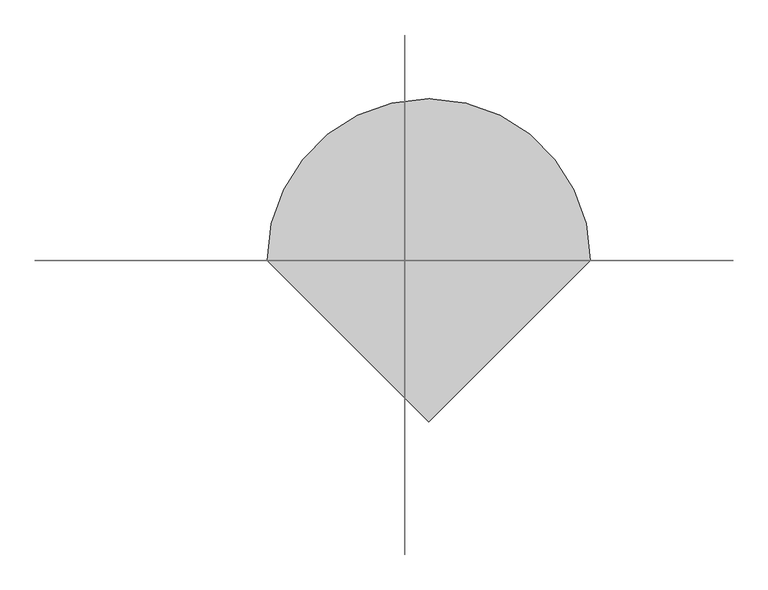
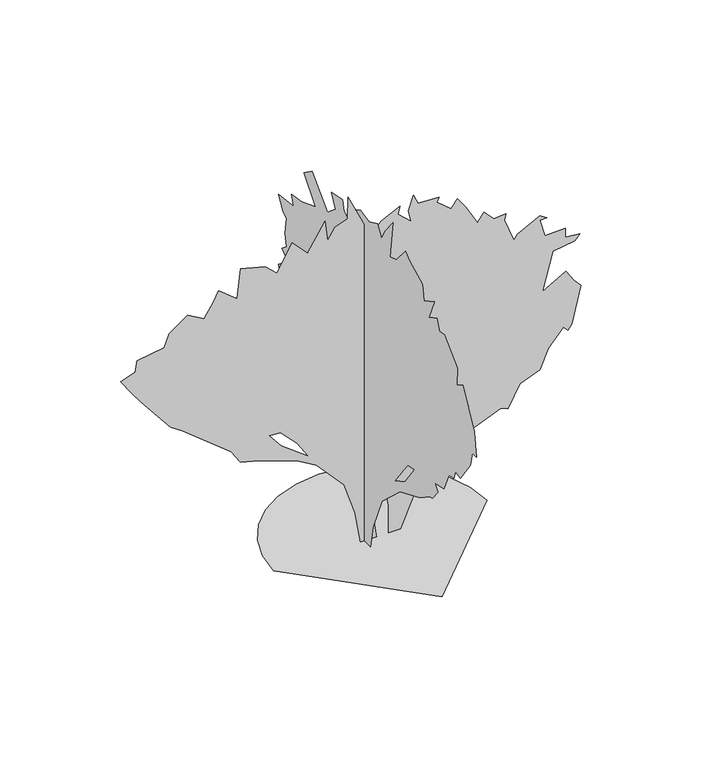
"""IFC4 building model written with IfcOpenShell, lengths in millimetres: proxy geometry, honey myrtle 26117 : honey myrtle 26117."""

from ifc_helpers import new_model, si_unit, origin, place, context, project, spatial, triangles, source, transform, mapped, element, save


def entourage_3ce3a2b3(model_context):
    return source(origin(), model_context, "Body", "Tessellation", [
        triangles([(-396.3767504, 0.0, 8.22e-05), (-385.8992649, 90.8237077, 8.22e-05), (-356.0543206, 174.2306261, 8.22e-05), (-309.2370838, 247.8313661, 8.22e-05), (-247.8313661, 309.2370838, 8.22e-05), (-174.2306261, 356.0543206, 8.22e-05), (-90.8237077, 385.8992649, 8.22e-05), (1.73e-05, 396.3767504, 8.22e-05), (90.8237077, 385.8992649, 8.22e-05), (174.2306261, 356.0543206, 8.22e-05), (247.8313661, 309.2370838, 8.22e-05), (309.2370838, 247.8313661, 8.22e-05), (356.0543206, 174.2306261, 8.22e-05), (385.8992649, 90.8237077, 8.22e-05), (396.3767504, -3.47e-05, 8.22e-05), (-5.2e-05, -396.3767504, 8.22e-05), (-59.3577095, 35.0059915, 9.26e-05), (-59.3577095, 44.8705806, 101.5460546), (-59.3577095, 75.4742449, 222.0478563), (-59.3577095, 168.9964434, 326.3007588), (-59.3577095, 285.8741748, 405.6706235), (-59.3579639, 459.2340692, 576.3228888), (-59.3579639, 503.9253456, 625.6344137), (-59.3579639, 553.1479589, 751.1941189), (-59.3579639, 491.6190474, 799.7715317), (-59.3579639, 530.478485, 828.915465), (-59.3579639, 501.3320083, 851.5849388), (-59.3579639, 511.0474763, 900.1598808), (-59.3579639, 501.3320083, 961.688756), (-59.3579639, 524.0014821, 977.8812269), (-59.3579639, 553.1479589, 1026.4561689), (-59.3579639, 455.9955677, 1039.4101748), (-59.3579639, 469.4956884, 1077.0376745), (-59.3579639, 404.1821606, 1087.9850441), (-59.3579639, 313.5068087, 1123.6085238), (-59.3579639, 387.9896896, 1211.0454105), (-59.3579639, 336.1762825, 1249.9048119), (-59.3579639, 235.7859349, 1149.5164627), (-59.3579639, 183.9712561, 1191.6144018), (-59.3579639, 209.8784683, 1243.4278816), (-59.3579639, 138.9198272, 1256.3183739), (-59.3579639, 128.9188388, 1217.5224134), (-59.3579639, 70.6279291, 1185.1373989), (-59.3579639, 83.5816624, 1253.143277), (-59.3579639, 25.4436618, 1284.1769932), (-59.3579639, -29.761912, 1272.5743584), (-59.3579639, -86.0073592, 1299.3586246), (-59.3579639, -110.7212849, 1256.3817421), (-59.3579639, -133.3899957, 1298.4822247), (-59.3579639, -185.2039207, 1363.2496376), (-59.3577095, -165.7739475, 1217.5224134), (-59.3577095, -207.8728858, 1230.4738758), (-59.3577095, -266.3644464, 1299.9199276), (-59.3577095, -292.0717617, 1279.0512886), (-59.3577095, -376.2676217, 1236.950806), (-59.3577095, -385.9830897, 1178.660396), (-59.3577095, -450.7505027, 1214.2838757), (-59.3577095, -418.3680679, 1133.3239918), (-59.3577095, -466.9429736, 1159.22946), (-59.3577095, -484.2835213, 1117.1086298), (-59.3577095, -515.5204227, 1123.6085238), (-59.3577095, -599.7162646, 1042.6486399), (-59.3577095, -596.4777632, 974.6427618), (-59.3577095, -635.3397079, 997.3122356), (-59.3577095, -709.8225889, 858.0619417), (-59.3577095, -722.7765947, 767.3865898), (-59.3577095, -696.8686558, 767.3865898), (-59.3577095, -683.91465, 712.3346449), (-59.3577095, -619.147237, 621.659293), (-59.3577095, -586.7622588, 628.1362959), (-59.3577095, -577.0493342, 595.7513177), (-59.3577095, -544.664356, 589.2743148), (-59.3577095, -512.2819213, 514.7914338), (-59.3577095, -453.9890041, 501.8400078), (-59.3577095, -473.4199765, 479.1705339), (-59.3577095, -438.083507, 433.2245012), (-59.3577095, -424.8450708, 430.5955919), (-59.3577095, -359.671251, 388.3935531), (-59.3577095, -230.5626891, 332.9860339), (-59.3577095, -112.6590482, 224.7923109), (-59.3577095, -55.1474106, 87.2636415), (-59.3577095, -39.476642, 8.38e-05), (-59.3577095, 5.8605105, 135.9018064), (-59.3577095, 2.7896791, 186.1833303), (-59.3577095, 12.337225, 304.2967785), (-59.3577095, 38.2442317, 288.1068329), (-59.3577095, 54.4362076, 262.1988576), (-59.3577095, 151.5875587, 349.6357444), (-59.3577095, 177.4947618, 469.4550296), (-59.3577095, 258.4549001, 547.176412), (-59.3577095, 255.2163986, 508.3169744), (-59.3577095, 226.0704487, 394.9721486), (-59.3577095, 255.2163986, 404.687653), (-59.3577095, 297.3143196, 550.4149135), (-59.3577095, 337.517407, 606.5056758), (-59.3577095, 326.4607781, 505.0785092), (-59.3577095, 307.0298058, 462.9780267), (-59.3577095, 358.8432129, 501.8400078), (-59.3579639, 368.5587173, 641.0903017), (-59.3579639, 410.6591635, 689.6651711), (-59.3579639, 410.6591635, 628.1362959), (-59.3577095, -198.157654, 356.112711), (-59.3577095, -261.769596, 391.7057055), (-59.3577095, -324.4541782, 475.9320325), (-59.3577095, -282.3562755, 469.4550296), (-59.3577095, -253.2100531, 430.5955919), (-267.2940953, -2.61e-05, 404.687653), (-308.6096875, -2.21e-05, 471.3142911), (-370.9208914, -1.84e-05, 534.2224425), (-413.0213739, -1.82e-05, 537.4609076), (-368.4215527, -2.15e-05, 482.1804156), (30.6369404, -5.02e-05, 0.0), (31.1304627, -4.38e-05, 108.1619844), (9.0696959, -3.61e-05, 237.4841779), (-47.0839311, -3.05e-05, 330.2047357), (-39.4309189, -4.01e-05, 170.4041154), (-14.7000316, -5.02e-05, 0.0), (-72.990889, -5.02e-05, 0.0), (-92.9872747, -4.29e-05, 122.5858678), (-134.4006626, -3.55e-05, 247.1552083), (-236.0793036, -2.88e-05, 358.7517941), (-302.2063538, -2.64e-05, 398.8659516), (-451.8807753, -2.32e-05, 453.2625587), (-519.8892331, -2.22e-05, 469.4550296), (-555.510133, -1.89e-05, 524.5069382), (-736.858366, -1.03e-05, 670.234235), (-778.9587759, -8.5e-06, 699.3807117), (-889.0625931, -4e-07, 835.3924679), (-924.6860727, 2.5e-06, 883.9674099), (-965.6003632, 6e-06, 942.4685629), (-911.7320669, 7.1e-06, 961.688756), (-905.255064, 9.6e-06, 1003.7892385), (-804.8642441, 1.06e-05, 1019.979166), (-785.4357788, 1.35e-05, 1068.5565788), (-717.4299007, 1.64e-05, 1117.1315208), (-655.8984821, 1.43e-05, 1081.5105846), (-620.2775459, 1.75e-05, 1136.5625296), (-600.8465735, 1.97e-05, 1172.1833931), (-532.8406591, 1.64e-05, 1117.1315208), (-519.8892331, 2.31e-05, 1230.4738758), (-429.2138449, 2.18e-05, 1207.8068727), (-383.8748972, 1.93e-05, 1165.7064629), (-328.8229886, 2.53e-05, 1266.0972828), (-270.5325967, 2.16e-05, 1204.5684076), (-205.7644389, 2.78e-05, 1308.1951492), (-196.0496976, 2.29e-05, 1227.2378815), (-167.6639666, 2.55e-05, 1270.8241745), (-121.5665623, 2.66e-05, 1288.7668293), (-119.7654549, 3.15e-05, 1371.5986919), (-34.1304544, 2.06e-05, 1188.3759367), (2.3015577, 2.34e-05, 1235.4267712), (72.7363851, 2.54e-05, 1269.3357479), (66.2596456, 2.37e-05, 1240.1892712), (114.8353143, 2.1e-05, 1194.8529396), (105.1200825, 2.37e-05, 1240.1892712), (124.5505553, 2.7e-05, 1295.2437595), (140.7425266, 2.47e-05, 1256.3817421), (218.4636638, 2.45e-05, 1253.143277), (211.1367854, 2.35e-05, 1235.7950626), (263.8015941, 2.08e-05, 1191.6144018), (286.4685245, 2.27e-05, 1223.9994164), (318.8535027, 2e-05, 1178.660396), (360.9514054, 1.56e-05, 1104.177515), (385.0814006, 1.75e-05, 1135.7446289), (422.4828604, 1.52e-05, 1097.7005121), (467.8192646, 1.54e-05, 1100.9390499), (461.3422617, 1.41e-05, 1078.2721195), (496.9657413, 8.7e-06, 987.5967676), (509.9172037, 9.8e-06, 1007.0277037), (594.1155527, 1.23e-05, 1049.1256428), (620.0235643, 1.14e-05, 1032.9331718), (593.290058, 1.13e-05, 1031.1069025), (613.5465614, 7.3e-06, 964.9272211), (688.0294424, 7.5e-06, 968.1657589), (688.0294424, 5.4e-06, 932.5448227), (743.0813147, 5e-06, 926.0678198), (723.6503786, 3.8e-06, 906.6368837), (642.6904947, 3.1e-06, 893.6828779), (603.8310571, -5.6e-06, 747.9555811), (691.2679075, -2.7e-06, 796.5330666), (720.4118408, -5.4e-06, 751.1941189), (746.3198524, -7.2e-06, 722.0501856), (713.9348379, -1.55e-05, 582.7973482), (697.7449104, -1.66e-05, 563.3688829), (681.5524395, -1.57e-05, 579.5613902), (626.5005672, -1.93e-05, 518.0299353), (594.1155527, -2.38e-05, 443.5470543), (519.6326717, -2.55e-05, 414.403121), (474.2962675, -3.03e-05, 333.4432371), (448.3882922, -2.98e-05, 343.1587415), (311.7719945, -3.3e-05, 288.0331637), (205.1723602, -3.7e-05, 221.2502851), (125.3034072, -4.32e-05, 117.1220752), (75.9746277, -5.02e-05, 0.0), (30.6369404, -3.34e-05, 281.62983), (43.5909303, -2.72e-05, 385.2566442), (7.9686832, -2.28e-05, 459.7395252), (-30.8919575, -2.45e-05, 430.5955919), (-38.6976243, -2.72e-05, 386.112624), (-2.6646859, -3.14e-05, 315.8842435), (150.4575132, -3.75e-05, 213.6229345), (215.0437962, -3.57e-05, 242.9182394), (296.5269221, -3.01e-05, 337.5199505), (331.8074721, -2.65e-05, 398.2106501), (278.0814637, -2.79e-05, 375.0661689), (195.3344433, -3.11e-05, 320.3901821), (154.7673882, -3.52e-05, 251.8887493)], [[16, 15, 1], [15, 14, 1], [1, 14, 2], [14, 13, 2], [2, 13, 3], [3, 13, 4], [13, 12, 4], [12, 11, 4], [4, 11, 5], [5, 11, 6], [6, 11, 7], [7, 11, 8], [8, 11, 9], [9, 11, 10], [90, 93, 91], [91, 93, 92], [93, 90, 94], [98, 95, 99], [17, 83, 18], [95, 98, 96], [50, 49, 51], [57, 56, 58], [85, 88, 86], [49, 48, 51], [84, 102, 85], [18, 83, 19], [83, 87, 19], [31, 30, 32], [19, 87, 20], [40, 39, 41], [41, 39, 42], [26, 25, 27], [30, 29, 32], [17, 82, 83], [82, 81, 83], [81, 80, 83], [83, 80, 84], [84, 80, 102], [80, 79, 102], [102, 79, 103], [79, 78, 103], [103, 78, 104], [78, 77, 104], [33, 32, 34], [66, 65, 67], [59, 58, 60], [36, 35, 37], [37, 35, 38], [86, 88, 87], [87, 88, 20], [88, 92, 20], [20, 92, 21], [92, 93, 21], [93, 97, 21], [21, 97, 22], [64, 63, 65], [53, 52, 54], [47, 46, 48], [75, 74, 76], [24, 23, 25], [44, 43, 45], [45, 43, 46], [96, 98, 97], [97, 98, 22], [98, 101, 22], [22, 101, 23], [23, 101, 25], [101, 100, 25], [69, 68, 70], [76, 74, 77], [77, 74, 104], [71, 70, 72], [88, 85, 89], [85, 102, 89], [102, 106, 89], [106, 105, 89], [54, 52, 55], [55, 52, 56], [61, 60, 62], [62, 60, 63], [42, 39, 43], [73, 72, 74], [46, 43, 48], [48, 43, 51], [65, 63, 67], [94, 90, 95], [89, 105, 90], [39, 38, 43], [67, 63, 68], [68, 63, 70], [70, 63, 72], [63, 60, 72], [60, 58, 72], [72, 58, 74], [74, 58, 104], [104, 58, 105], [105, 58, 90], [58, 56, 90], [56, 52, 90], [52, 51, 90], [51, 43, 90], [43, 38, 90], [90, 38, 95], [95, 38, 99], [99, 38, 100], [38, 35, 100], [100, 35, 25], [25, 35, 27], [35, 34, 27], [34, 32, 27], [32, 29, 27], [29, 28, 27], [112, 196, 113], [197, 196, 201], [196, 195, 113], [113, 195, 114], [149, 148, 150], [196, 112, 201], [171, 170, 172], [201, 207, 197], [145, 144, 146], [156, 155, 157], [176, 175, 177], [177, 175, 178], [152, 151, 153], [112, 194, 201], [194, 193, 201], [193, 192, 201], [201, 192, 202], [192, 191, 202], [202, 191, 203], [114, 195, 115], [195, 200, 115], [200, 199, 115], [170, 169, 172], [207, 206, 197], [158, 157, 159], [166, 165, 167], [161, 160, 162], [143, 142, 144], [130, 129, 131], [117, 116, 118], [118, 116, 119], [119, 116, 120], [116, 115, 120], [115, 107, 120], [120, 107, 121], [121, 107, 122], [107, 111, 122], [122, 111, 123], [111, 110, 123], [138, 137, 139], [115, 199, 107], [164, 163, 165], [140, 139, 141], [184, 183, 185], [191, 190, 203], [203, 190, 204], [174, 173, 175], [175, 173, 178], [172, 169, 173], [180, 179, 181], [199, 198, 107], [141, 139, 142], [189, 188, 190], [123, 110, 124], [124, 110, 125], [169, 168, 173], [155, 154, 157], [157, 154, 159], [132, 131, 133], [183, 182, 185], [190, 188, 204], [148, 147, 150], [147, 146, 150], [206, 205, 197], [137, 136, 139], [182, 181, 185], [181, 179, 185], [185, 179, 186], [135, 134, 136], [107, 198, 108], [159, 154, 160], [134, 133, 136], [173, 168, 178], [178, 168, 179], [131, 129, 133], [129, 128, 133], [128, 127, 133], [133, 127, 136], [127, 126, 136], [136, 126, 139], [126, 125, 139], [125, 110, 139], [139, 110, 142], [110, 109, 142], [142, 109, 144], [144, 109, 146], [146, 109, 150], [109, 108, 150], [108, 198, 150], [198, 197, 150], [197, 205, 150], [205, 204, 150], [204, 188, 150], [188, 187, 150], [187, 186, 150], [186, 179, 150], [179, 168, 150], [168, 167, 150], [151, 150, 153], [153, 150, 154], [162, 160, 163], [160, 154, 163], [154, 150, 163], [150, 167, 163], [163, 167, 165]], closed=False),
    ])


if __name__ == "__main__":
    model = new_model("IFC4")
    model_context = context("Model", 3, world=origin())
    ifc_project = project(units=[si_unit("LENGTHUNIT", "METRE", prefix="MILLI")], contexts=[model_context])
    site = spatial("IfcSite", under=ifc_project)
    building = spatial("IfcBuilding", under=site)
    placement = place(None, origin())
    entourage_shape = entourage_3ce3a2b3(model_context)
    element("IfcBuildingElementProxy", 1, Name="honey myrtle 26117 : honey myrtle 26117", ObjectType="honey myrtle 26117 : honey myrtle 26117", at=placement, inside=building, context=model_context, shape_type="MappedRepresentation", body=[
        mapped(entourage_shape, transform((0.0, 0.0, 0.0), x_axis=(1.0, 0.0, 0.0), y_axis=(0.0, 1.0, 0.0), z_axis=(0.0, 0.0, 1.0))),
    ])
    save(model, "model.ifc")

# Revit data of these elements
# Type "honey myrtle 26117 : honey myrtle 26117"
#   built-in parameter 1005195 = "RPC-16-G3GK-N2Q0-PN0G-6000-ST1L-LVER-AU"
#   Height = 0
